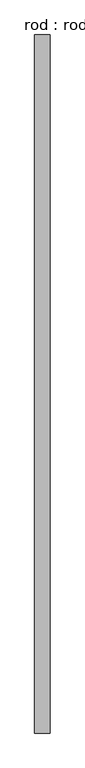
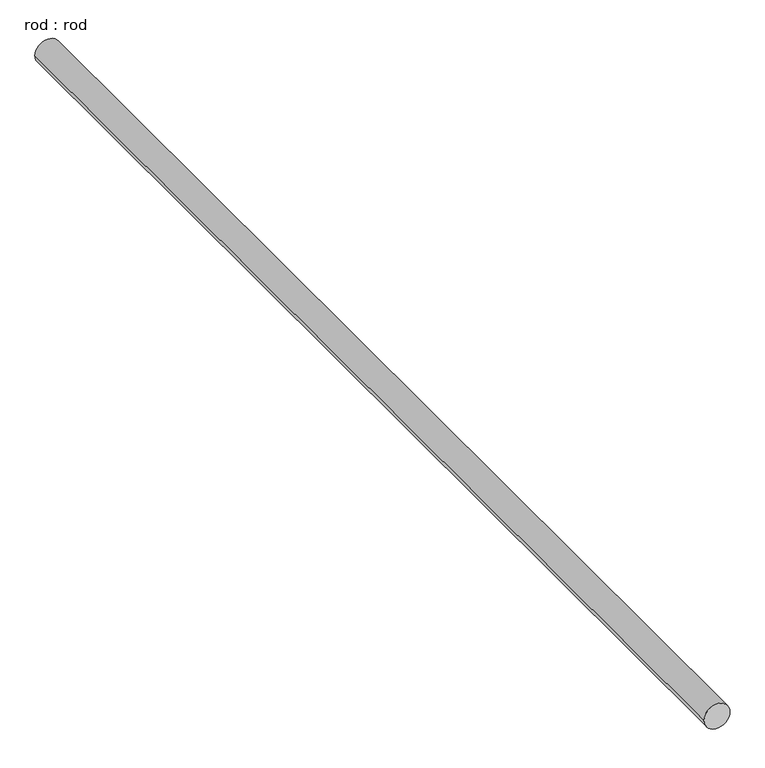
"""IFC4 building model written with IfcOpenShell, lengths in millimetres: proxy geometry, rod : rod."""

from ifc_helpers import new_model, si_unit, point, frame, frame_2d, origin, place, context, project, spatial, circle_curve, trimmed, segment, composite_curve, outline, extrude, source, transform, mapped, element, save


def rod_rod_95acf935(model_context):
    return source(origin(), model_context, "Body", "SweptSolid", [
        extrude(outline(composite_curve([segment(trimmed(circle_curve(frame_2d((0.0108462, 0.0)), 200.0), [point((0.0108462, 200.0))], [point((0.0108462, -200.0))], False, "CARTESIAN"), True, "CONTINUOUS"), segment(trimmed(circle_curve(frame_2d((0.0108462, 0.0)), 200.0), [point((0.0108462, -200.0))], [point((0.0108462, 200.0))], False, "CARTESIAN"), True, "CONTINUOUS")], self_intersect=False)), frame((0.0, -4879.4936069, 0.0), z_axis=(0.0, 1.0, 0.0), x_axis=(0.0, 0.0, 1.0)), (0.0, 0.0, 1.0), 17944.4444444),
    ])


if __name__ == "__main__":
    model = new_model("IFC4")
    model_context = context("Model", 3, world=origin())
    ifc_project = project(units=[si_unit("LENGTHUNIT", "METRE", prefix="MILLI")], contexts=[model_context])
    site = spatial("IfcSite", under=ifc_project)
    building = spatial("IfcBuilding", under=site)
    placement = place(None, origin())
    rod_rod_shape = rod_rod_95acf935(model_context)
    element("IfcBuildingElementProxy", 1, Name="rod : rod", ObjectType="rod : rod", at=placement, inside=building, context=model_context, shape_type="MappedRepresentation", body=[
        mapped(rod_rod_shape, transform((0.0, 0.0, 0.0), x_axis=(1.0, 0.0, 0.0), y_axis=(0.0, 1.0, 0.0), z_axis=(0.0, 0.0, 1.0))),
    ])
    save(model, "model.ifc")

# Revit data of these elements
# Type "rod : rod"
#   Default Elevation = 0
